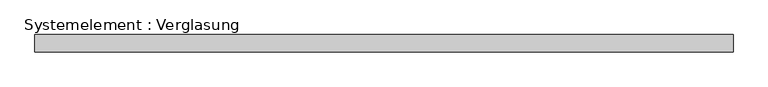
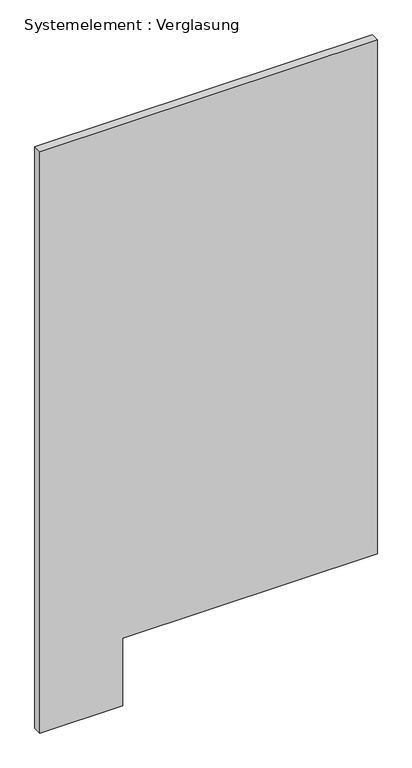
"""IFC4 building model written with IfcOpenShell, lengths in millimetres: plate geometry, Systemelement : Verglasung."""

import ifcopenshell
import ifcopenshell.guid

model = None  # the IFC model being written
_history = None  # IfcOwnerHistory: only IFC2X3 demands one
_inside = {}  # id of a spatial element -> (the spatial element, [elements in it])
_under = {}  # id of a project, library or spatial element -> (it, [spatial elements below it])
_declared = {}  # id of a project -> (the project, [libraries it declares])
_typed = {}  # id of a type object -> (the type object, [elements of that type])
_made_of = {}  # id of a material, layer set ... -> (it, [elements and type objects made of it])


def new_model(schema):
    """Start an empty IFC model of exactly this schema.

    Asked for "IFC4X3", IfcOpenShell would pick the latest addendum, in which some entities
    have other attributes; the version numbers below select the first issue.
    IFC2X3 requires an IfcOwnerHistory on every rooted entity: one is made here for all.
    """
    global model, _history
    if schema == "IFC4X3":
        model = ifcopenshell.file(schema_version=(4, 3, 0, 0))
    else:
        model = ifcopenshell.file(schema=schema)
    _inside.clear()
    _under.clear()
    _declared.clear()
    _typed.clear()
    _made_of.clear()
    _history = None
    if model.schema == "IFC2X3":
        org = make("IfcOrganization", Name="unknown")
        user = make(
            "IfcPersonAndOrganization",
            ThePerson=make("IfcPerson", FamilyName="unknown"),
            TheOrganization=org,
        )
        app = make(
            "IfcApplication",
            ApplicationDeveloper=org,
            Version="unknown",
            ApplicationFullName="unknown",
            ApplicationIdentifier="unknown",
        )
        _history = make(
            "IfcOwnerHistory",
            OwningUser=user,
            OwningApplication=app,
            ChangeAction="ADDED",
            CreationDate=0,
        )
    return model


def make(cls, **values):
    """One entity of the class cls with the attributes given. An attribute that is None is left unset."""
    return model.create_entity(
        cls, **{name: value for name, value in values.items() if value is not None}
    )


def rooted(cls, **values):
    """An entity with a GlobalId (a new one), such as an element, a storey or a relation."""
    return make(cls, GlobalId=ifcopenshell.guid.new(), OwnerHistory=_history, **values)


def si_unit(unit_type, name, prefix=None):
    """IfcSIUnit, for example si_unit("LENGTHUNIT", "METRE", prefix="MILLI")."""
    return make("IfcSIUnit", UnitType=unit_type, Prefix=prefix, Name=name)


def assignment(units):
    """IfcUnitAssignment: the units of a project."""
    return None if units is None else make("IfcUnitAssignment", Units=units)


def point(xyz):
    """IfcCartesianPoint."""
    return None if xyz is None else make("IfcCartesianPoint", Coordinates=xyz)


def direction(xyz):
    """IfcDirection."""
    return None if xyz is None else make("IfcDirection", DirectionRatios=xyz)


def frame(location, z_axis=None, x_axis=None):
    """IfcAxis2Placement3D, a coordinate frame: its origin and axes. An axis left out is left unset."""
    return make(
        "IfcAxis2Placement3D",
        Location=point(location),
        Axis=direction(z_axis),
        RefDirection=direction(x_axis),
    )


def origin():
    """The frame at (0, 0, 0) with its axes left unset."""
    return frame((0.0, 0.0, 0.0))


def place(relative_to, where):
    """IfcLocalPlacement: puts the frame where relative to a parent placement (None: the world)."""
    return make(
        "IfcLocalPlacement", PlacementRelTo=relative_to, RelativePlacement=where
    )


def context(
    kind, dimensions, precision=None, world=None, true_north=None, identifier=None
):
    """IfcGeometricRepresentationContext, for example the 3D "Model" context."""
    return make(
        "IfcGeometricRepresentationContext",
        ContextIdentifier=identifier,
        ContextType=kind,
        CoordinateSpaceDimension=dimensions,
        Precision=precision,
        WorldCoordinateSystem=world,
        TrueNorth=true_north,
    )


def project(units=None, contexts=None):
    """IfcProject with its units and contexts."""
    return rooted(
        "IfcProject",
        Name="project",
        RepresentationContexts=contexts,
        UnitsInContext=assignment(units),
    )


def spatial(cls, under=None, at=None, **own):
    """A site, building, storey or space (cls), placed at a placement, below another one or the project."""
    s = rooted(cls, ObjectPlacement=at, **own)
    if under is not None:
        _under.setdefault(under.id(), (under, []))[1].append(s)
    return s


def polyline(points):
    """IfcPolyline through the points."""
    return make("IfcPolyline", Points=[point(p) for p in points])


def outline(outer, holes=None, kind="AREA"):
    """IfcArbitraryClosedProfileDef: a profile drawn as a closed curve; with holes, ...WithVoids."""
    if holes is None:
        return make("IfcArbitraryClosedProfileDef", ProfileType=kind, OuterCurve=outer)
    return make(
        "IfcArbitraryProfileDefWithVoids",
        ProfileType=kind,
        OuterCurve=outer,
        InnerCurves=holes,
    )


def extrude(swept, where, along, depth):
    """IfcExtrudedAreaSolid: the profile swept, set in the frame where, extruded along a direction by depth."""
    return make(
        "IfcExtrudedAreaSolid",
        SweptArea=swept,
        Position=where,
        ExtrudedDirection=direction(along),
        Depth=depth,
    )


def shape(context_of_items, identifier, shape_type, items):
    """IfcShapeRepresentation: the items that make up one representation, for example the "Body"."""
    return make(
        "IfcShapeRepresentation",
        ContextOfItems=context_of_items,
        RepresentationIdentifier=identifier,
        RepresentationType=shape_type,
        Items=items,
    )


def source(mapping_origin, context_of_items, identifier, shape_type, items):
    """IfcRepresentationMap: a shape defined once, which mapped items show again and again."""
    return make(
        "IfcRepresentationMap",
        MappingOrigin=mapping_origin,
        MappedRepresentation=shape(context_of_items, identifier, shape_type, items),
    )


def transform(
    local_origin,
    x_axis=None,
    y_axis=None,
    z_axis=None,
    scale=None,
    scale2=None,
    scale3=None,
    uniform=True,
):
    """IfcCartesianTransformationOperator3D, or its non-uniform kind. x_axis, y_axis, z_axis: its Axis1, 2, 3."""
    if uniform:
        return make(
            "IfcCartesianTransformationOperator3D",
            Axis1=direction(x_axis),
            Axis2=direction(y_axis),
            LocalOrigin=point(local_origin),
            Scale=scale,
            Axis3=direction(z_axis),
        )
    return make(
        "IfcCartesianTransformationOperator3DnonUniform",
        Axis1=direction(x_axis),
        Axis2=direction(y_axis),
        LocalOrigin=point(local_origin),
        Scale=scale,
        Axis3=direction(z_axis),
        Scale2=scale2,
        Scale3=scale3,
    )


def mapped(mapping_source, mapping_target):
    """IfcMappedItem: shows the shape of a source again, moved by a transform."""
    return make(
        "IfcMappedItem", MappingSource=mapping_source, MappingTarget=mapping_target
    )


def made_of(thing, what):
    """Note that an element or type object is made of a material, layer set ...; save() writes the relation."""
    if what is not None:
        _made_of.setdefault(what.id(), (what, []))[1].append(thing)
    return thing


def element(
    cls,
    number,
    at=None,
    inside=None,
    cuts=None,
    type_object=None,
    material=None,
    context=None,
    identifier="Body",
    shape_type=None,
    held_by="IfcProductDefinitionShape",
    body=None,
    shapes=None,
    **own,
):
    """One element of the class cls, such as IfcWall. Its Tag is "e" and its number.

    at: its placement. inside: the storey or other place that contains it. cuts: it is an
    opening in that element (IfcRelVoidsElement). A single representation is given by context,
    identifier, shape_type and body (its items); several are given by shapes. held_by: the class
    of the entity that holds the representations. save() writes the other relations.
    """
    e = rooted(cls, Tag="e%d" % number, ObjectPlacement=at, **own)
    if body is not None:
        shapes = [shape(context, identifier, shape_type, body)]
    if shapes is not None:
        e.Representation = make(held_by, Representations=shapes)
    if inside is not None:
        _inside.setdefault(inside.id(), (inside, []))[1].append(e)
    if cuts is not None:
        rooted(
            "IfcRelVoidsElement", RelatingBuildingElement=cuts, RelatedOpeningElement=e
        )
    if type_object is not None:
        _typed.setdefault(type_object.id(), (type_object, []))[1].append(e)
    return made_of(e, material)


def aggregate(whole, parts):
    """IfcRelAggregates: a whole, such as a stair, and the parts it consists of."""
    return rooted("IfcRelAggregates", RelatingObject=whole, RelatedObjects=parts)


def save(model, path):
    """Write the relations noted so far, then the file.

    IfcRelAggregates (storeys below a building ...), IfcRelContainedInSpatialStructure (elements
    in a storey), IfcRelDefinesByType, IfcRelAssociatesMaterial and IfcRelDeclares: one each for
    every whole, place, type object, material and project.
    """
    for whole, parts in _under.values():
        aggregate(whole, parts)
    for where, things in _inside.values():
        rooted(
            "IfcRelContainedInSpatialStructure",
            RelatedElements=things,
            RelatingStructure=where,
        )
    for kind, things in _typed.values():
        rooted("IfcRelDefinesByType", RelatedObjects=things, RelatingType=kind)
    for what, things in _made_of.values():
        rooted("IfcRelAssociatesMaterial", RelatedObjects=things, RelatingMaterial=what)
    for by, libraries in _declared.values():
        rooted("IfcRelDeclares", RelatingContext=by, RelatedDefinitions=libraries)
    model.write(path)


def systemelement_verglasung_406041e1(model_context):
    return source(origin(), model_context, "Body", "SweptSolid", [
        extrude(outline(polyline([(0.0, -610.0), (0.0, -310.6220396), (257.7235772, -310.6220396), (257.7235772, 610.0), (2220.0, 610.0), (2220.0, -610.0), (0.0, -610.0)])), frame((0.0, -15.0, 0.0), z_axis=(0.0, 1.0, 0.0), x_axis=(0.0, 0.0, 1.0)), (0.0, 0.0, 1.0), 30.0),
    ])


if __name__ == "__main__":
    model = new_model("IFC4")
    model_context = context("Model", 3, world=origin())
    ifc_project = project(units=[si_unit("LENGTHUNIT", "METRE", prefix="MILLI")], contexts=[model_context])
    site = spatial("IfcSite", under=ifc_project)
    building = spatial("IfcBuilding", under=site)
    placement = place(None, origin())
    systemelement_verglasung_shape = systemelement_verglasung_406041e1(model_context)
    element("IfcPlate", 1, ObjectType="Systemelement : Verglasung", at=placement, inside=building, context=model_context, shape_type="MappedRepresentation", body=[
        mapped(systemelement_verglasung_shape, transform((0.0, 0.0, 0.0), x_axis=(1.0, 0.0, 0.0), y_axis=(0.0, 1.0, 0.0), z_axis=(0.0, 0.0, 1.0))),
    ])
    save(model, "model.ifc")

# Revit data of these elements
# Type "Systemelement : Verglasung"
#   Construction Type Id = "GSP4R"
#   Analytic Construction = "1/8 Zoll Pilkington-Verglasung einfach"
#   Visual Light Transmittance = 0.9
#   Solar Heat Gain Coefficient = 0.86
#   Heat Transfer Coefficient (U) = 6.7069 W/(m²·K)
# Element 1 (IfcPlate, "Systemelement : Verglasung")
#   Materials on its faces: "Glas"
# Materials
#   "Glas": class "Glas", colour RGB 0 0 255, transparency 0.75, Comments = "Render-Darstellung nicht aktualisiert ", Cost = 0
